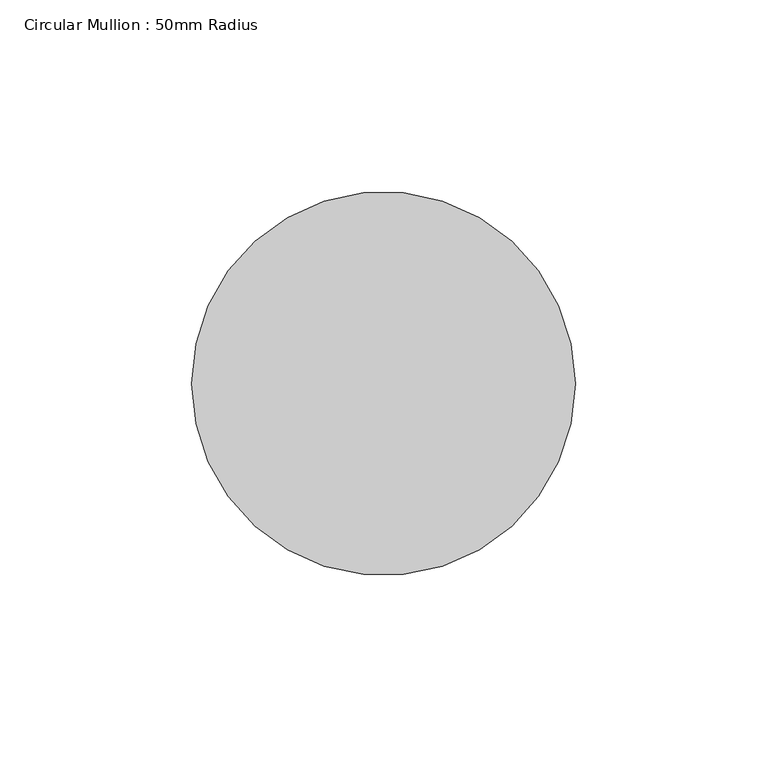
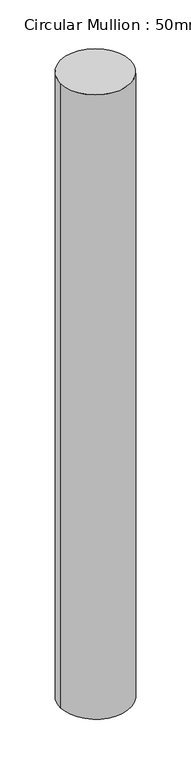
"""IFC4 building model written with IfcOpenShell, lengths in millimetres: member geometry, Circular Mullion : 50mm Radius."""

from ifc_helpers import new_model, si_unit, point, frame, origin, origin_2d, place, context, project, spatial, circle_curve, trimmed, segment, composite_curve, outline, extrude, source, transform, mapped, element, save


def circular_mullion_50mm_radius_54281050(model_context):
    return source(origin(), model_context, "Body", "SweptSolid", [
        extrude(outline(composite_curve([segment(trimmed(circle_curve(origin_2d(), 50.0), [point((50.0, 0.0))], [point((-50.0, 0.0))], False, "CARTESIAN"), True, "CONTINUOUS"), segment(trimmed(circle_curve(origin_2d(), 50.0), [point((-50.0, 0.0))], [point((50.0, 0.0))], False, "CARTESIAN"), True, "CONTINUOUS")], self_intersect=False)), frame((0.0, 0.0, -945.4279901), z_axis=(0.0, 0.0, 1.0), x_axis=(1.0, 0.0, 0.0)), (0.0, 0.0, 1.0), 945.4279901),
    ])


if __name__ == "__main__":
    model = new_model("IFC4")
    model_context = context("Model", 3, world=origin())
    ifc_project = project(units=[si_unit("LENGTHUNIT", "METRE", prefix="MILLI")], contexts=[model_context])
    site = spatial("IfcSite", under=ifc_project)
    building = spatial("IfcBuilding", under=site)
    placement = place(None, origin())
    circular_mullion_50mm_radius_shape = circular_mullion_50mm_radius_54281050(model_context)
    element("IfcMember", 1, ObjectType="Circular Mullion : 50mm Radius", at=placement, inside=building, context=model_context, shape_type="MappedRepresentation", body=[
        mapped(circular_mullion_50mm_radius_shape, transform((0.0, 0.0, 0.0), x_axis=(1.0, 0.0, 0.0), y_axis=(0.0, 1.0, 0.0), z_axis=(0.0, 0.0, 1.0))),
    ])
    save(model, "model.ifc")

# Revit data of these elements
# Type "Circular Mullion : 50mm Radius"
#   built-in parameter 1007350 = 0.164042 (stored number, unit not read)
# Element 1 (IfcMember, "Circular Mullion : 50mm Radius")
#   Materials on its faces: "Aluminium"
# Materials
#   "Aluminium": class "Metal", colour RGB 247 247 247, transparency 0, Description = "Aluminium 6061", Cost = 0
